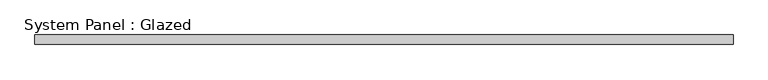
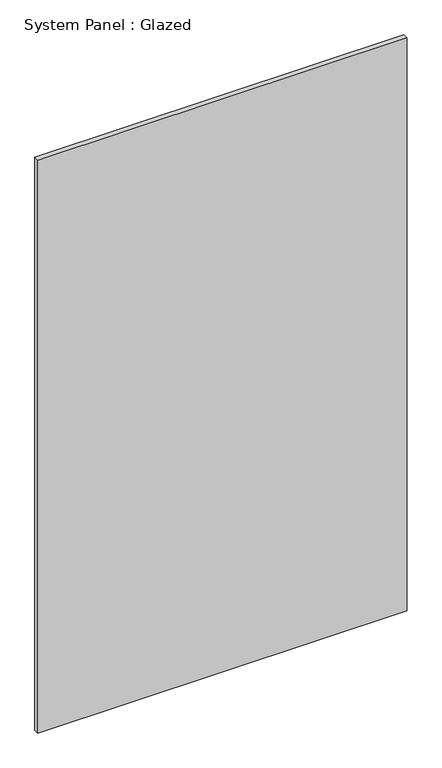
"""IFC4 building model written with IfcOpenShell, lengths in millimetres: plate geometry, System Panel : Glazed."""

from ifc_helpers import new_model, si_unit, origin, origin_with_axes, place, context, project, spatial, polyline, outline, extrude, source, transform, mapped, element, save


def system_panel_glazed_1b9f2f65(model_context):
    return source(origin(), model_context, "Body", "SweptSolid", [
        extrude(outline(polyline([(915.0000002, 24.5), (-915.0000002, 24.5), (-915.0000002, 49.5), (915.0000002, 49.5), (915.0000002, 24.5)])), origin_with_axes(), (0.0, 0.0, 1.0), 3000.0),
    ])


if __name__ == "__main__":
    model = new_model("IFC4")
    model_context = context("Model", 3, world=origin())
    ifc_project = project(units=[si_unit("LENGTHUNIT", "METRE", prefix="MILLI")], contexts=[model_context])
    site = spatial("IfcSite", under=ifc_project)
    building = spatial("IfcBuilding", under=site)
    placement = place(None, origin())
    system_panel_glazed_shape = system_panel_glazed_1b9f2f65(model_context)
    element("IfcPlate", 1, ObjectType="System Panel : Glazed", at=placement, inside=building, context=model_context, shape_type="MappedRepresentation", body=[
        mapped(system_panel_glazed_shape, transform((0.0, 0.0, 0.0), x_axis=(1.0, 0.0, 0.0), y_axis=(0.0, 1.0, 0.0), z_axis=(0.0, 0.0, 1.0))),
    ])
    save(model, "model.ifc")

# Revit data of these elements
# Type "System Panel : Glazed"
#   Construction Type Id = "GSP4R"
#   Analytic Construction = "1/8 in Pilkington single glazing"
#   Visual Light Transmittance = 0.9
#   Solar Heat Gain Coefficient = 0.86
#   Heat Transfer Coefficient (U) = 6.7069 W/(m²·K)
#   Define Thermal Properties by = 1
# Element 1 (IfcPlate, "System Panel : Glazed")
#   Materials on its faces: "Glass"
# Materials
#   "Glass": class "Glass", colour RGB 0 128 192, transparency 0.9, Description = "Soda Lime Glass", Cost = 0
